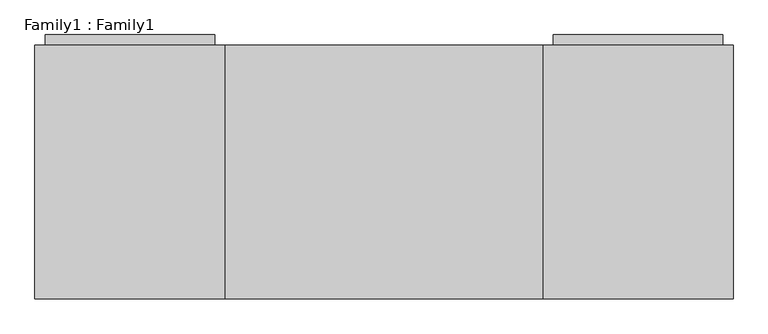
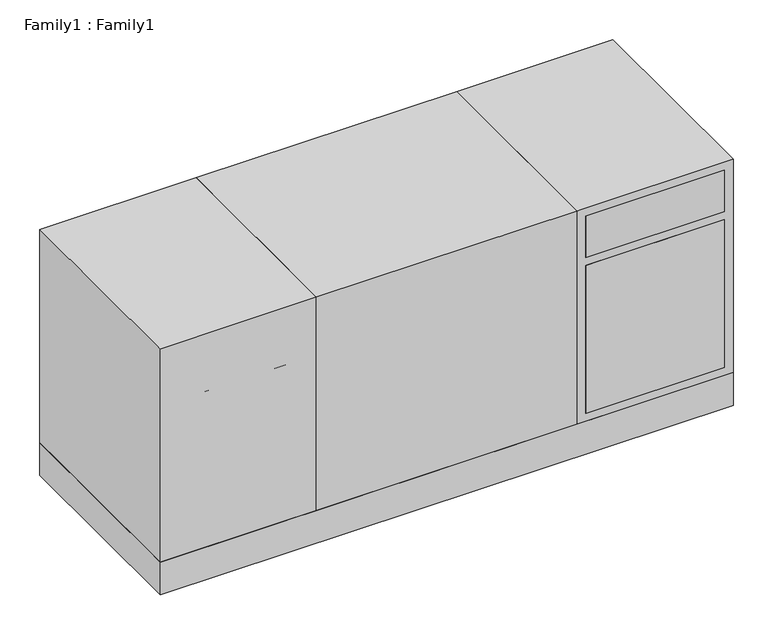
"""IFC4 building model written with IfcOpenShell, lengths in millimetres: proxy geometry, Family1 : Family1."""

from ifc_helpers import new_model, si_unit, frame, origin, place, context, project, spatial, polyline, outline, extrude, source, transform, mapped, element, save


def family1_family1_84e39cff(model_context):
    return source(origin(), model_context, "Body", "SweptSolid", [
        extrude(outline(polyline([(-1447.8, 660.4), (228.6, 660.4), (228.6, 50.8), (-1447.8, 50.8), (-1447.8, 660.4)])), frame((0.0, 0.0, 1082.3221517), z_axis=(0.0, 0.0, 1.0), x_axis=(1.0, 0.0, 0.0)), (0.0, 0.0, 1.0), 101.6),
        extrude(outline(polyline([(-990.6, 660.4), (-228.6, 660.4), (-228.6, 50.8), (-990.6, 50.8), (-990.6, 660.4)])), frame((0.0, 0.0, 1183.9221517), z_axis=(0.0, 0.0, 1.0), x_axis=(1.0, 0.0, 0.0)), (0.0, 0.0, 1.0), 660.4),
        extrude(outline(polyline([(-1447.8, 660.4), (-990.6, 660.4), (-990.6, 50.8), (-1447.8, 50.8), (-1447.8, 660.4)])), frame((0.0, 0.0, 1183.9221517), z_axis=(0.0, 0.0, 1.0), x_axis=(1.0, 0.0, 0.0)), (0.0, 0.0, 1.0), 660.4),
        extrude(outline(polyline([(-1422.4, 685.8), (-1016.0, 685.8), (-1016.0, 50.8), (-1422.4, 50.8), (-1422.4, 685.8)])), frame((0.0, 0.0, 1691.9221517), z_axis=(0.0, 0.0, 1.0), x_axis=(1.0, 0.0, 0.0)), (0.0, 0.0, 1.0), 127.0),
        extrude(outline(polyline([(-1422.4, 685.8), (-1016.0, 685.8), (-1016.0, 50.8), (-1422.4, 50.8), (-1422.4, 685.8)])), frame((0.0, 0.0, 1209.3221517), z_axis=(0.0, 0.0, 1.0), x_axis=(1.0, 0.0, 0.0)), (0.0, 0.0, 1.0), 457.2),
        extrude(outline(polyline([(-203.2, 685.8), (203.2, 685.8), (203.2, 50.8), (-203.2, 50.8), (-203.2, 685.8)])), frame((0.0, 0.0, 1691.9221517), z_axis=(0.0, 0.0, 1.0), x_axis=(1.0, 0.0, 0.0)), (0.0, 0.0, 1.0), 127.0),
        extrude(outline(polyline([(-203.2, 685.8), (203.2, 685.8), (203.2, 50.8), (-203.2, 50.8), (-203.2, 685.8)])), frame((0.0, 0.0, 1209.3221517), z_axis=(0.0, 0.0, 1.0), x_axis=(1.0, 0.0, 0.0)), (0.0, 0.0, 1.0), 457.2),
        extrude(outline(polyline([(-228.6, 660.4), (228.6, 660.4), (228.6, 50.8), (-228.6, 50.8), (-228.6, 660.4)])), frame((0.0, 0.0, 1183.9221517), z_axis=(0.0, 0.0, 1.0), x_axis=(1.0, 0.0, 0.0)), (0.0, 0.0, 1.0), 660.4),
    ])


if __name__ == "__main__":
    model = new_model("IFC4")
    model_context = context("Model", 3, world=origin())
    ifc_project = project(units=[si_unit("LENGTHUNIT", "METRE", prefix="MILLI")], contexts=[model_context])
    site = spatial("IfcSite", under=ifc_project)
    building = spatial("IfcBuilding", under=site)
    placement = place(None, origin())
    family1_family1_shape = family1_family1_84e39cff(model_context)
    element("IfcBuildingElementProxy", 1, Name="Family1 : Family1", ObjectType="Family1 : Family1", at=placement, inside=building, context=model_context, shape_type="MappedRepresentation", body=[
        mapped(family1_family1_shape, transform((0.0, 0.0, 0.0), x_axis=(1.0, 0.0, 0.0), y_axis=(0.0, 1.0, 0.0), z_axis=(0.0, 0.0, 1.0))),
    ])
    save(model, "model.ifc")

# Revit data of these elements
# Type "Family1 : Family1"
#   top gas surface = 0' - 4"
#   stove area = 2' - 6"
#   side small cupboard = 0' - 10"
#   middle strip = 0' - 1"
#   left box half = 0' - 8"
#   drawers depth = 2' - 1"
#   cabinet height = 2' - 6"
#   cabinet depth = 2' - 0"
#   bottom strip = 0' - 4"
#   Default Elevation = 0
